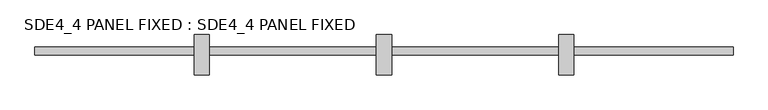
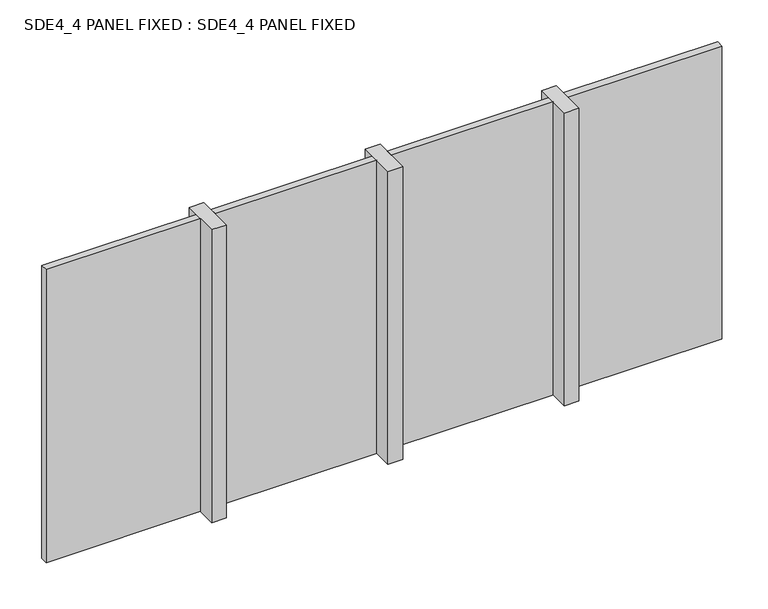
"""IFC4 building model written with IfcOpenShell, lengths in millimetres: plate geometry, SDE4_4 PANEL FIXED : SDE4_4 PANEL FIXED."""

import ifcopenshell
import ifcopenshell.guid

model = None  # the IFC model being written
_history = None  # IfcOwnerHistory: only IFC2X3 demands one
_inside = {}  # id of a spatial element -> (the spatial element, [elements in it])
_under = {}  # id of a project, library or spatial element -> (it, [spatial elements below it])
_declared = {}  # id of a project -> (the project, [libraries it declares])
_typed = {}  # id of a type object -> (the type object, [elements of that type])
_made_of = {}  # id of a material, layer set ... -> (it, [elements and type objects made of it])


def new_model(schema):
    """Start an empty IFC model of exactly this schema.

    Asked for "IFC4X3", IfcOpenShell would pick the latest addendum, in which some entities
    have other attributes; the version numbers below select the first issue.
    IFC2X3 requires an IfcOwnerHistory on every rooted entity: one is made here for all.
    """
    global model, _history
    if schema == "IFC4X3":
        model = ifcopenshell.file(schema_version=(4, 3, 0, 0))
    else:
        model = ifcopenshell.file(schema=schema)
    _inside.clear()
    _under.clear()
    _declared.clear()
    _typed.clear()
    _made_of.clear()
    _history = None
    if model.schema == "IFC2X3":
        org = make("IfcOrganization", Name="unknown")
        user = make(
            "IfcPersonAndOrganization",
            ThePerson=make("IfcPerson", FamilyName="unknown"),
            TheOrganization=org,
        )
        app = make(
            "IfcApplication",
            ApplicationDeveloper=org,
            Version="unknown",
            ApplicationFullName="unknown",
            ApplicationIdentifier="unknown",
        )
        _history = make(
            "IfcOwnerHistory",
            OwningUser=user,
            OwningApplication=app,
            ChangeAction="ADDED",
            CreationDate=0,
        )
    return model


def make(cls, **values):
    """One entity of the class cls with the attributes given. An attribute that is None is left unset."""
    return model.create_entity(
        cls, **{name: value for name, value in values.items() if value is not None}
    )


def rooted(cls, **values):
    """An entity with a GlobalId (a new one), such as an element, a storey or a relation."""
    return make(cls, GlobalId=ifcopenshell.guid.new(), OwnerHistory=_history, **values)


def si_unit(unit_type, name, prefix=None):
    """IfcSIUnit, for example si_unit("LENGTHUNIT", "METRE", prefix="MILLI")."""
    return make("IfcSIUnit", UnitType=unit_type, Prefix=prefix, Name=name)


def assignment(units):
    """IfcUnitAssignment: the units of a project."""
    return None if units is None else make("IfcUnitAssignment", Units=units)


def point(xyz):
    """IfcCartesianPoint."""
    return None if xyz is None else make("IfcCartesianPoint", Coordinates=xyz)


def direction(xyz):
    """IfcDirection."""
    return None if xyz is None else make("IfcDirection", DirectionRatios=xyz)


def frame(location, z_axis=None, x_axis=None):
    """IfcAxis2Placement3D, a coordinate frame: its origin and axes. An axis left out is left unset."""
    return make(
        "IfcAxis2Placement3D",
        Location=point(location),
        Axis=direction(z_axis),
        RefDirection=direction(x_axis),
    )


def origin():
    """The frame at (0, 0, 0) with its axes left unset."""
    return frame((0.0, 0.0, 0.0))


def origin_with_axes():
    """The frame at (0, 0, 0) with the z axis (0, 0, 1) and the x axis (1, 0, 0) written out."""
    return frame((0.0, 0.0, 0.0), z_axis=(0.0, 0.0, 1.0), x_axis=(1.0, 0.0, 0.0))


def place(relative_to, where):
    """IfcLocalPlacement: puts the frame where relative to a parent placement (None: the world)."""
    return make(
        "IfcLocalPlacement", PlacementRelTo=relative_to, RelativePlacement=where
    )


def context(
    kind, dimensions, precision=None, world=None, true_north=None, identifier=None
):
    """IfcGeometricRepresentationContext, for example the 3D "Model" context."""
    return make(
        "IfcGeometricRepresentationContext",
        ContextIdentifier=identifier,
        ContextType=kind,
        CoordinateSpaceDimension=dimensions,
        Precision=precision,
        WorldCoordinateSystem=world,
        TrueNorth=true_north,
    )


def project(units=None, contexts=None):
    """IfcProject with its units and contexts."""
    return rooted(
        "IfcProject",
        Name="project",
        RepresentationContexts=contexts,
        UnitsInContext=assignment(units),
    )


def spatial(cls, under=None, at=None, **own):
    """A site, building, storey or space (cls), placed at a placement, below another one or the project."""
    s = rooted(cls, ObjectPlacement=at, **own)
    if under is not None:
        _under.setdefault(under.id(), (under, []))[1].append(s)
    return s


def polyline(points):
    """IfcPolyline through the points."""
    return make("IfcPolyline", Points=[point(p) for p in points])


def outline(outer, holes=None, kind="AREA"):
    """IfcArbitraryClosedProfileDef: a profile drawn as a closed curve; with holes, ...WithVoids."""
    if holes is None:
        return make("IfcArbitraryClosedProfileDef", ProfileType=kind, OuterCurve=outer)
    return make(
        "IfcArbitraryProfileDefWithVoids",
        ProfileType=kind,
        OuterCurve=outer,
        InnerCurves=holes,
    )


def extrude(swept, where, along, depth):
    """IfcExtrudedAreaSolid: the profile swept, set in the frame where, extruded along a direction by depth."""
    return make(
        "IfcExtrudedAreaSolid",
        SweptArea=swept,
        Position=where,
        ExtrudedDirection=direction(along),
        Depth=depth,
    )


def shape(context_of_items, identifier, shape_type, items):
    """IfcShapeRepresentation: the items that make up one representation, for example the "Body"."""
    return make(
        "IfcShapeRepresentation",
        ContextOfItems=context_of_items,
        RepresentationIdentifier=identifier,
        RepresentationType=shape_type,
        Items=items,
    )


def source(mapping_origin, context_of_items, identifier, shape_type, items):
    """IfcRepresentationMap: a shape defined once, which mapped items show again and again."""
    return make(
        "IfcRepresentationMap",
        MappingOrigin=mapping_origin,
        MappedRepresentation=shape(context_of_items, identifier, shape_type, items),
    )


def transform(
    local_origin,
    x_axis=None,
    y_axis=None,
    z_axis=None,
    scale=None,
    scale2=None,
    scale3=None,
    uniform=True,
):
    """IfcCartesianTransformationOperator3D, or its non-uniform kind. x_axis, y_axis, z_axis: its Axis1, 2, 3."""
    if uniform:
        return make(
            "IfcCartesianTransformationOperator3D",
            Axis1=direction(x_axis),
            Axis2=direction(y_axis),
            LocalOrigin=point(local_origin),
            Scale=scale,
            Axis3=direction(z_axis),
        )
    return make(
        "IfcCartesianTransformationOperator3DnonUniform",
        Axis1=direction(x_axis),
        Axis2=direction(y_axis),
        LocalOrigin=point(local_origin),
        Scale=scale,
        Axis3=direction(z_axis),
        Scale2=scale2,
        Scale3=scale3,
    )


def mapped(mapping_source, mapping_target):
    """IfcMappedItem: shows the shape of a source again, moved by a transform."""
    return make(
        "IfcMappedItem", MappingSource=mapping_source, MappingTarget=mapping_target
    )


def made_of(thing, what):
    """Note that an element or type object is made of a material, layer set ...; save() writes the relation."""
    if what is not None:
        _made_of.setdefault(what.id(), (what, []))[1].append(thing)
    return thing


def element(
    cls,
    number,
    at=None,
    inside=None,
    cuts=None,
    type_object=None,
    material=None,
    context=None,
    identifier="Body",
    shape_type=None,
    held_by="IfcProductDefinitionShape",
    body=None,
    shapes=None,
    **own,
):
    """One element of the class cls, such as IfcWall. Its Tag is "e" and its number.

    at: its placement. inside: the storey or other place that contains it. cuts: it is an
    opening in that element (IfcRelVoidsElement). A single representation is given by context,
    identifier, shape_type and body (its items); several are given by shapes. held_by: the class
    of the entity that holds the representations. save() writes the other relations.
    """
    e = rooted(cls, Tag="e%d" % number, ObjectPlacement=at, **own)
    if body is not None:
        shapes = [shape(context, identifier, shape_type, body)]
    if shapes is not None:
        e.Representation = make(held_by, Representations=shapes)
    if inside is not None:
        _inside.setdefault(inside.id(), (inside, []))[1].append(e)
    if cuts is not None:
        rooted(
            "IfcRelVoidsElement", RelatingBuildingElement=cuts, RelatedOpeningElement=e
        )
    if type_object is not None:
        _typed.setdefault(type_object.id(), (type_object, []))[1].append(e)
    return made_of(e, material)


def aggregate(whole, parts):
    """IfcRelAggregates: a whole, such as a stair, and the parts it consists of."""
    return rooted("IfcRelAggregates", RelatingObject=whole, RelatedObjects=parts)


def save(model, path):
    """Write the relations noted so far, then the file.

    IfcRelAggregates (storeys below a building ...), IfcRelContainedInSpatialStructure (elements
    in a storey), IfcRelDefinesByType, IfcRelAssociatesMaterial and IfcRelDeclares: one each for
    every whole, place, type object, material and project.
    """
    for whole, parts in _under.values():
        aggregate(whole, parts)
    for where, things in _inside.values():
        rooted(
            "IfcRelContainedInSpatialStructure",
            RelatedElements=things,
            RelatingStructure=where,
        )
    for kind, things in _typed.values():
        rooted("IfcRelDefinesByType", RelatedObjects=things, RelatingType=kind)
    for what, things in _made_of.values():
        rooted("IfcRelAssociatesMaterial", RelatedObjects=things, RelatingMaterial=what)
    for by, libraries in _declared.values():
        rooted("IfcRelDeclares", RelatingContext=by, RelatedDefinitions=libraries)
    model.write(path)


def sde4_4_panel_fixed_sde4_4_panel_fixed_1951d40c(model_context):
    return source(origin(), model_context, "Body", "SweptSolid", [
        extrude(outline(polyline([(-1150.0, 132.5), (-1150.0, -132.5), (-1250.0, -132.5), (-1250.0, 132.5), (-1150.0, 132.5)])), origin_with_axes(), (0.0, 0.0, 1.0), 2109.5956314),
        extrude(outline(polyline([(50.0, 132.5), (50.0, -132.5), (-50.0, -132.5), (-50.0, 132.5), (50.0, 132.5)])), origin_with_axes(), (0.0, 0.0, 1.0), 2109.5956314),
        extrude(outline(polyline([(1250.0, 132.5), (1250.0, -132.5), (1150.0, -132.5), (1150.0, 132.5), (1250.0, 132.5)])), origin_with_axes(), (0.0, 0.0, 1.0), 2109.5956314),
        extrude(outline(polyline([(2299.0, 50.0), (2299.0, 0.0), (1250.0, 0.0), (1250.0, 50.0), (2299.0, 50.0)])), origin_with_axes(), (0.0, 0.0, 1.0), 2109.5956314),
        extrude(outline(polyline([(1150.0, 50.0), (1150.0, 0.0), (50.0, 0.0), (50.0, 50.0), (1150.0, 50.0)])), origin_with_axes(), (0.0, 0.0, 1.0), 2109.5956314),
        extrude(outline(polyline([(-50.0, 50.0), (-50.0, 0.0), (-1150.0, 0.0), (-1150.0, 50.0), (-50.0, 50.0)])), origin_with_axes(), (0.0, 0.0, 1.0), 2109.5956314),
        extrude(outline(polyline([(-1250.0, 50.0), (-1250.0, 0.0), (-2300.0, 0.0), (-2300.0, 50.0), (-1250.0, 50.0)])), origin_with_axes(), (0.0, 0.0, 1.0), 2109.5956314),
    ])


if __name__ == "__main__":
    model = new_model("IFC4")
    model_context = context("Model", 3, world=origin())
    ifc_project = project(units=[si_unit("LENGTHUNIT", "METRE", prefix="MILLI")], contexts=[model_context])
    site = spatial("IfcSite", under=ifc_project)
    building = spatial("IfcBuilding", under=site)
    placement = place(None, origin())
    sde4_4_panel_fixed_sde4_4_panel_fixed_shape = sde4_4_panel_fixed_sde4_4_panel_fixed_1951d40c(model_context)
    element("IfcPlate", 1, ObjectType="SDE4_4 PANEL FIXED : SDE4_4 PANEL FIXED", at=placement, inside=building, context=model_context, shape_type="MappedRepresentation", body=[
        mapped(sde4_4_panel_fixed_sde4_4_panel_fixed_shape, transform((0.0, 0.0, 0.0), x_axis=(1.0, 0.0, 0.0), y_axis=(0.0, 1.0, 0.0), z_axis=(0.0, 0.0, 1.0))),
    ])
    save(model, "model.ifc")

# Revit data of these elements
# Type "SDE4_4 PANEL FIXED : SDE4_4 PANEL FIXED"
#   Type Mark = "CW-GLASS"
#   Analytic Construction = "<None>"
#   Glass = Glass
#   Frame = Aluminium
# Element 1 (IfcPlate, "SDE4_4 PANEL FIXED : SDE4_4 PANEL FIXED")
#   Materials on its faces: "Glass", "Aluminium"
# Materials
#   "Glass": class "Glass", colour RGB 0 128 192, transparency 0.9, Keynote = "L40", Cost = 0
#   "Aluminium": class "Unassigned", colour RGB 247 247 247, transparency 0, Cost = 0
